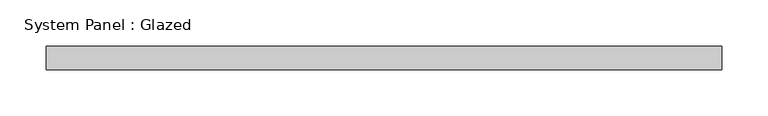
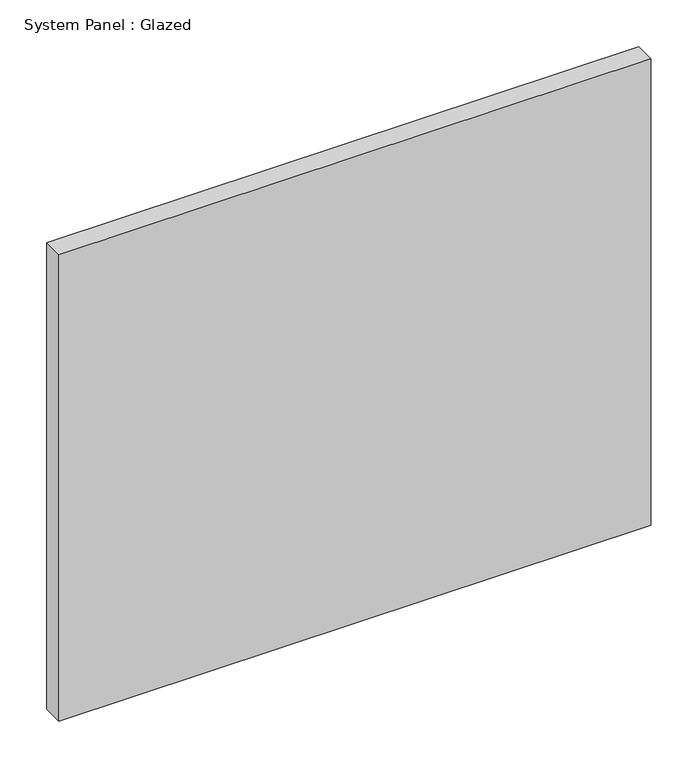
"""IFC4 building model written with IfcOpenShell, lengths in millimetres: plate geometry, System Panel : Glazed."""

from ifc_helpers import new_model, si_unit, origin, origin_with_axes, place, context, project, spatial, polyline, outline, extrude, source, transform, mapped, element, save


def system_panel_glazed_164c7573(model_context):
    return source(origin(), model_context, "Body", "SweptSolid", [
        extrude(outline(polyline([(365.9255071, 19.05), (-365.9255071, 19.05), (-365.9255071, 44.45), (365.9255071, 44.45), (365.9255071, 19.05)])), origin_with_axes(), (0.0, 0.0, 1.0), 609.6),
    ])


if __name__ == "__main__":
    model = new_model("IFC4")
    model_context = context("Model", 3, world=origin())
    ifc_project = project(units=[si_unit("LENGTHUNIT", "METRE", prefix="MILLI")], contexts=[model_context])
    site = spatial("IfcSite", under=ifc_project)
    building = spatial("IfcBuilding", under=site)
    placement = place(None, origin())
    system_panel_glazed_shape = system_panel_glazed_164c7573(model_context)
    element("IfcPlate", 1, ObjectType="System Panel : Glazed", at=placement, inside=building, context=model_context, shape_type="MappedRepresentation", body=[
        mapped(system_panel_glazed_shape, transform((0.0, 0.0, 0.0), x_axis=(1.0, 0.0, 0.0), y_axis=(0.0, 1.0, 0.0), z_axis=(0.0, 0.0, 1.0))),
    ])
    save(model, "model.ifc")

# Revit data of these elements
# Element 1 (IfcPlate, "System Panel : Glazed")
#   Materials on its faces: "Glass"
# Materials
#   "Glass": class "Glass", colour RGB 0 128 192, transparency 0.75
